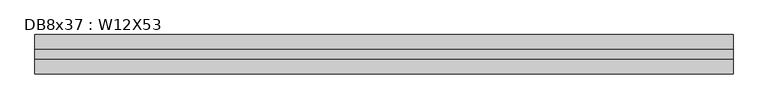
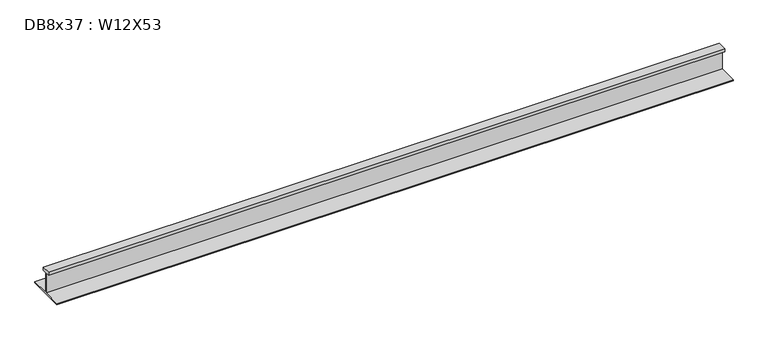
"""IFC4 building model written with IfcOpenShell, lengths in millimetres: beam geometry, DB8x37 : W12X53."""

from ifc_helpers import new_model, si_unit, frame, origin, place, context, project, spatial, polyline, outline, extrude, source, transform, mapped, element, save


def db8x37_w12x53_c6cfd1d7(model_context):
    return source(origin(), model_context, "Body", "SweptSolid", [
        extrude(outline(polyline([(38.1, 145.415), (38.1, 120.015), (2.921, 120.015), (2.921, -48.4505), (152.4, -48.4505), (152.4, -58.1025), (-152.4, -58.1025), (-152.4, -48.4505), (-2.921, -48.4505), (-2.921, 120.015), (-38.1, 120.015), (-38.1, 145.415), (38.1, 145.415)])), frame((-2705.1, 0.0, 0.0), z_axis=(1.0, 0.0, 0.0), x_axis=(0.0, 1.0, 0.0)), (0.0, 0.0, 1.0), 5413.629),
    ])


if __name__ == "__main__":
    model = new_model("IFC4")
    model_context = context("Model", 3, world=origin())
    ifc_project = project(units=[si_unit("LENGTHUNIT", "METRE", prefix="MILLI")], contexts=[model_context])
    site = spatial("IfcSite", under=ifc_project)
    building = spatial("IfcBuilding", under=site)
    placement = place(None, origin())
    db8x37_w12x53_shape = db8x37_w12x53_c6cfd1d7(model_context)
    element("IfcBeam", 1, ObjectType="DB8x37 : W12X53", at=placement, inside=building, context=model_context, shape_type="MappedRepresentation", body=[
        mapped(db8x37_w12x53_shape, transform((0.0, 0.0, 0.0), x_axis=(1.0, 0.0, 0.0), y_axis=(0.0, 1.0, 0.0), z_axis=(0.0, 0.0, 1.0))),
    ])
    save(model, "model.ifc")

# Revit data of these elements
# Type "DB8x37 : W12X53"
#   Assembly Code = "B10"
#   W = 53
#   Length [instance default] = 5' - 0"
#   bf = 0' - 10"
#   d = 1' - 0.1"
#   k = 0' - 1 3/8"
#   k2 = 0' - 0.8"
#   tf = 0' - 0.575"
#   tw = 0' - 0.345"
#   A = 0.108333 SF
#   Structural Material [instance default] = Steel ASTM A992
# Element 1 (IfcBeam, "DB8x37 : W12X53")
#   Materials on its faces: "Steel ASTM A992"
# Materials
#   "Steel ASTM A992": class "Metal", colour RGB 199 199 199, transparency 0, Description = "Structural steel 50ksi", Cost = 0
